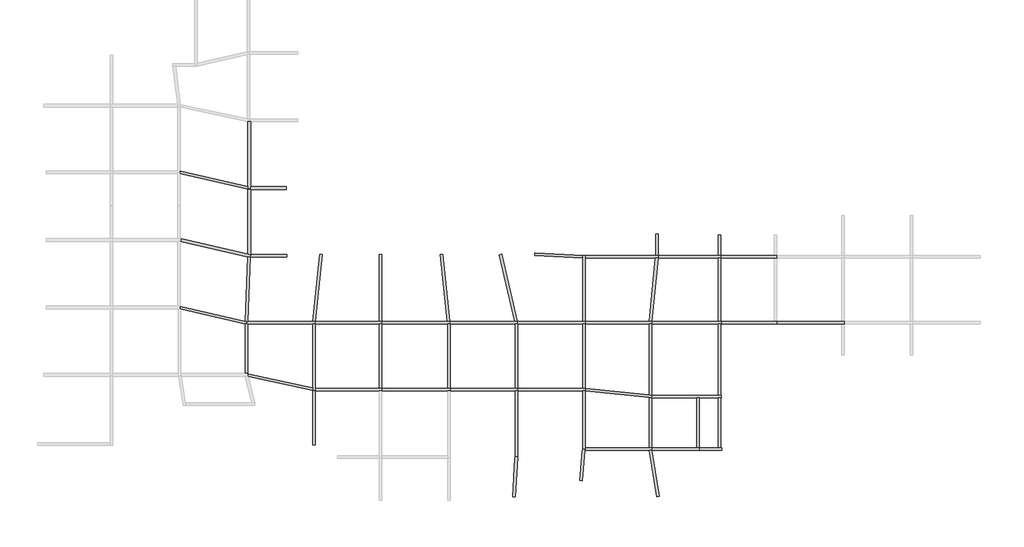
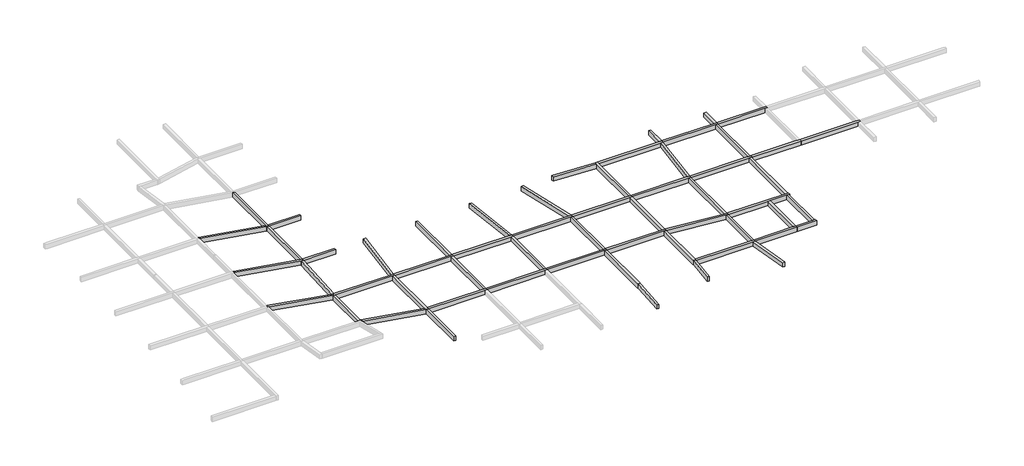
# One storey, part 4 of 8: 57 beams.
"""IFC4 building model written with IfcOpenShell, lengths in millimetres."""

from ifc_helpers import new_model, si_unit, frame, origin, place, context, project, spatial, polyline, outline, extrude, faceted_brep, element, save

model = new_model("IFC4")

# Units and contexts
model_context = context("Model", 3, world=origin())
ifc_project = project(units=[si_unit("LENGTHUNIT", "METRE", prefix="MILLI")], contexts=[model_context])

# Site, building, storey
site = spatial("IfcSite", under=ifc_project)
building = spatial("IfcBuilding", under=site)
storey = spatial("IfcBuildingStorey", under=building, Name="层高", Elevation=3300.0)

# Beams
placement = place(None, origin())
element("IfcBeam", 1, ObjectType="混凝土 - 矩形梁 : KL_beam", at=placement, inside=storey, context=model_context, shape_type="Brep", body=[
    faceted_brep([(165142.8646968, 66807.9309409, 3300.0), (165142.8646968, 59204.3834573, 3300.0), (165142.8646968, 58896.7990062, 3300.0), (165442.8646968, 58896.7990062, 3300.0), (165442.8646968, 59166.6493896, 3300.0), (165442.8646968, 66779.3985459, 3300.0), (165277.0990615, 66779.3985459, 3300.0), (165142.8646968, 66807.9309409, 2700.0), (165142.8646968, 59204.3834573, 2700.0), (165142.8646968, 58896.7990062, 2700.0), (165277.0990615, 66779.3985459, 2700.0), (165442.8646968, 66779.3985459, 2700.0), (165442.8646968, 59166.6493896, 2700.0), (165442.8646968, 58896.7990062, 2700.0)], [[[0, 1, 2, 3, 4, 5, 6]], [[2, 1, 0, 7, 8, 9]], [[9, 8, 7, 10, 11, 12, 13]], [[3, 13, 12, 11, 5, 4]], [[0, 6, 10, 7]], [[6, 5, 11, 10]], [[3, 2, 9, 13]]]),
])
element("IfcBeam", 2, ObjectType="混凝土 - 矩形梁 : KL_beam", at=placement, inside=storey, context=model_context, shape_type="SweptSolid", body=[
    extrude(outline(polyline([(165142.8646968, 58896.7990062), (157226.4248507, 60688.1226811), (157226.4248507, 60995.7071323), (165142.8646968, 59204.3834573), (165142.8646968, 58896.7990062)])), frame((0.0, 0.0, 2700.0), z_axis=(0.0, 0.0, 1.0), x_axis=(1.0, 0.0, 0.0)), (0.0, 0.0, 1.0), 600.0),
])
element("IfcBeam", 3, ObjectType="混凝土 - 矩形梁 : KL_beam", at=placement, inside=storey, context=model_context, shape_type="Brep", body=[
    faceted_brep([(169649.165188, 59166.6493896, 3300.0), (169649.165188, 58866.6493896, 3300.0), (169649.165188, 58866.6493896, 2700.0), (169649.165188, 59166.6493896, 2700.0), (165442.8646968, 59166.6493896, 3300.0), (165442.8646968, 59136.4997731, 3300.0), (165442.8646968, 58896.7990062, 3300.0), (165142.8646968, 58896.7990062, 3300.0), (165142.8646968, 58866.6493896, 3300.0), (165442.8646968, 58866.6493896, 3300.0), (165142.8646968, 58866.6493896, 2700.0), (165442.8646968, 58866.6493896, 2700.0), (165142.8646968, 58896.7990062, 2700.0), (165442.8646968, 58896.7990062, 2700.0), (165442.8646968, 59136.4997731, 2700.0), (165442.8646968, 59166.6493896, 2700.0)], [[[0, 1, 2, 3]], [[1, 0, 4, 5, 6, 7, 8, 9]], [[2, 1, 9, 8, 10, 11]], [[3, 2, 11, 10, 12, 13, 14, 15]], [[0, 3, 15, 4]], [[10, 8, 7, 12]], [[13, 6, 5, 4, 15, 14]], [[6, 13, 12, 7]]]),
])
element("IfcBeam", 4, ObjectType="混凝土 - 矩形梁 : KL_beam", at=placement, inside=storey, context=model_context, shape_type="Brep", body=[
    faceted_brep([(165375.3793805, 50905.9465121, 3300.0), (165380.6883405, 50928.942144, 3300.0), (165442.8646968, 51198.2575315, 3300.0), (165142.8646968, 51267.5179888, 3300.0), (157280.5913749, 53082.6668088, 3300.0), (157246.4106924, 52782.6668088, 3300.0), (165137.4631911, 50960.8737924, 3300.0), (165275.7743556, 50928.942144, 3300.0), (165375.3793805, 50905.9465121, 2700.0), (157246.4106924, 52782.6668088, 2700.0), (165137.4631911, 50960.8737924, 2700.0), (165275.7743556, 50928.942144, 2700.0), (165442.8646968, 51198.2575315, 2700.0), (165380.6883405, 50928.942144, 2700.0), (157280.5913749, 53082.6668088, 2700.0), (165142.8646968, 51267.5179888, 2700.0)], [[[0, 1, 2, 3, 4, 5, 6, 7]], [[8, 0, 7, 6, 5, 9, 10, 11]], [[12, 13, 8, 11, 10, 9, 14, 15]], [[2, 12, 15, 14, 4, 3]], [[2, 1, 0, 8, 13, 12]], [[4, 14, 9, 5]]]),
])
element("IfcBeam", 5, ObjectType="混凝土 - 矩形梁 : KL_beam", at=placement, inside=storey, context=model_context, shape_type="Brep", body=[
    faceted_brep([(165442.8646968, 58866.6493896, 3300.0), (165142.8646968, 58866.6493896, 3300.0), (165142.8646968, 51267.5179888, 3300.0), (165442.8646968, 51198.2575315, 3300.0), (165442.8646968, 51228.942144, 3300.0), (165142.8646968, 58866.6493896, 2700.0), (165142.8646968, 51267.5179888, 2700.0), (165442.8646968, 58866.6493896, 2700.0), (165442.8646968, 51228.942144, 2700.0), (165442.8646968, 51198.2575315, 2700.0)], [[[0, 1, 2, 3, 4]], [[1, 5, 6, 2]], [[5, 7, 8, 9, 6]], [[7, 0, 4, 3, 9, 8]], [[1, 0, 7, 5]], [[3, 2, 6, 9]]]),
])
element("IfcBeam", 6, ObjectType="混凝土 - 矩形梁 : KL_beam", at=placement, inside=storey, context=model_context, shape_type="Brep", body=[
    faceted_brep([(169692.8646968, 51228.942144, 3300.0), (169692.8646968, 50928.942144, 3300.0), (169692.8646968, 50928.942144, 2700.0), (169692.8646968, 51228.942144, 2700.0), (165442.8646968, 51228.942144, 3300.0), (165442.8646968, 51198.2575315, 3300.0), (165380.6883405, 50928.942144, 3300.0), (165436.3392696, 50928.942144, 3300.0), (165380.6883405, 50928.942144, 2700.0), (165436.3392696, 50928.942144, 2700.0), (165442.8646968, 51198.2575315, 2700.0), (165442.8646968, 51228.942144, 2700.0)], [[[0, 1, 2, 3]], [[1, 0, 4, 5, 6, 7]], [[2, 1, 7, 6, 8, 9]], [[3, 2, 9, 8, 10, 11]], [[0, 3, 11, 4]], [[6, 5, 10, 8]], [[5, 4, 11, 10]]]),
    faceted_brep([(165136.0424839, 50928.942144, 2700.0), (165136.0424839, 50928.942144, 3300.0), (165137.4631911, 50960.8737924, 3300.0), (165137.4631911, 50960.8737924, 2700.0), (165275.7743556, 50928.942144, 3300.0), (165275.7743556, 50928.942144, 2700.0), (165142.8646968, 50959.6267565, 2700.0), (165142.8646968, 50959.6267565, 3300.0)], [[[0, 1, 2, 3]], [[4, 5, 6, 3, 2, 7]], [[1, 4, 7, 2]], [[1, 0, 5, 4]], [[5, 0, 3, 6]]]),
])
element("IfcBeam", 7, ObjectType="混凝土 - 矩形梁 : KL_beam", at=placement, inside=storey, context=model_context, shape_type="Brep", body=[
    faceted_brep([(164960.8749274, 43383.0583741, 3300.0), (164801.942538, 43419.7508073, 3300.0), (157226.4248507, 45168.6968726, 3300.0), (157165.9144091, 45182.6668088, 3300.0), (157131.7337266, 44882.6668088, 3300.0), (157298.8240678, 44844.090964, 3300.0), (164793.7845861, 43113.7429866, 3300.0), (164926.6942449, 43083.0583741, 3300.0), (157131.7337266, 44882.6668088, 2700.0), (157298.8240678, 44844.090964, 2700.0), (164793.7845861, 43113.7429866, 2700.0), (164926.6942449, 43083.0583741, 2700.0), (157165.9144091, 45182.6668088, 2700.0), (157226.4248507, 45168.6968726, 2700.0), (164801.942538, 43419.7508073, 2700.0), (164960.8749274, 43383.0583741, 2700.0)], [[[0, 1, 2, 3, 4, 5, 6, 7]], [[7, 6, 5, 4, 8, 9, 10, 11]], [[11, 10, 9, 8, 12, 13, 14, 15]], [[3, 2, 1, 0, 15, 14, 13, 12]], [[3, 12, 8, 4]], [[0, 7, 11, 15]]]),
])
element("IfcBeam", 8, ObjectType="混凝土 - 矩形梁 : KL_beam", at=placement, inside=storey, context=model_context, shape_type="Brep", body=[
    faceted_brep([(164960.8749274, 43383.0583741, 3300.0), (164926.6942449, 43083.0583741, 3300.0), (165093.7845861, 43083.0583741, 3300.0), (172693.7845861, 43083.0583741, 3300.0), (172978.8451928, 43083.0583741, 3300.0), (173010.3764633, 43383.0583741, 3300.0), (172708.7239795, 43383.0583741, 3300.0), (165100.606799, 43383.0583741, 3300.0), (164926.6942449, 43083.0583741, 2700.0), (165093.7845861, 43083.0583741, 2700.0), (172693.7845861, 43083.0583741, 2700.0), (172978.8451928, 43083.0583741, 2700.0), (164960.8749274, 43383.0583741, 2700.0), (165100.606799, 43383.0583741, 2700.0), (172708.7239795, 43383.0583741, 2700.0), (173010.3764633, 43383.0583741, 2700.0)], [[[0, 1, 2, 3, 4, 5, 6, 7]], [[1, 8, 9, 10, 11, 4, 3, 2]], [[8, 12, 13, 14, 15, 11, 10, 9]], [[12, 0, 7, 6, 5, 15, 14, 13]], [[0, 12, 8, 1]], [[5, 4, 11, 15]]]),
])
element("IfcBeam", 9, ObjectType="混凝土 - 矩形梁 : KL_beam", at=placement, inside=storey, context=model_context, shape_type="SweptSolid", body=[
    extrude(outline(polyline([(165275.7743556, 50928.942144), (165375.3793805, 50905.9465121), (165380.6883405, 50928.942144), (165436.3392696, 50928.942144), (165100.606799, 43383.0583741), (164960.8749274, 43383.0583741), (164801.942538, 43419.7508073), (165136.0424839, 50928.942144), (165275.7743556, 50928.942144)])), frame((0.0, 0.0, 2700.0), z_axis=(0.0, 0.0, 1.0), x_axis=(1.0, 0.0, 0.0)), (0.0, 0.0, 1.0), 600.0),
])
element("IfcBeam", 10, ObjectType="混凝土 - 矩形梁 : KL_beam", at=placement, inside=storey, context=model_context, shape_type="SweptSolid", body=[
    extrude(outline(polyline([(173536.3056367, 51256.9718763), (173834.6622053, 51225.6133373), (173010.3764633, 43383.0583741), (172708.7239795, 43383.0583741), (173536.3056367, 51256.9718763)])), frame((0.0, 0.0, 2700.0), z_axis=(0.0, 0.0, 1.0), x_axis=(1.0, 0.0, 0.0)), (0.0, 0.0, 1.0), 600.0),
])
element("IfcBeam", 11, ObjectType="混凝土 - 矩形梁 : KL_beam", at=placement, inside=storey, context=model_context, shape_type="Brep", body=[
    faceted_brep([(173010.3764633, 43383.0583741, 3300.0), (172978.8451928, 43083.0583741, 3300.0), (172993.7845861, 43083.0583741, 3300.0), (180493.7845861, 43083.0583741, 3300.0), (180793.7845861, 43083.0583741, 3300.0), (180793.7845861, 43383.0583741, 3300.0), (180493.7845861, 43383.0583741, 3300.0), (172978.8451928, 43083.0583741, 2700.0), (172993.7845861, 43083.0583741, 2700.0), (180493.7845861, 43083.0583741, 2700.0), (180793.7845861, 43083.0583741, 2700.0), (173010.3764633, 43383.0583741, 2700.0), (180493.7845861, 43383.0583741, 2700.0), (180793.7845861, 43383.0583741, 2700.0)], [[[0, 1, 2, 3, 4, 5, 6]], [[1, 7, 8, 9, 10, 4, 3, 2]], [[7, 11, 12, 13, 10, 9, 8]], [[11, 0, 6, 5, 13, 12]], [[1, 0, 11, 7]], [[5, 4, 10, 13]]]),
])
element("IfcBeam", 12, ObjectType="混凝土 - 矩形梁 : KL_beam", at=placement, inside=storey, context=model_context, shape_type="Brep", body=[
    faceted_brep([(188778.8451928, 43083.0583741, 3300.0), (188778.8451928, 43383.0583741, 3300.0), (188477.1927089, 43383.0583741, 3300.0), (180793.7845861, 43383.0583741, 3300.0), (180793.7845861, 43083.0583741, 3300.0), (188493.7845861, 43083.0583741, 3300.0), (188778.8451928, 43083.0583741, 2700.0), (180793.7845861, 43083.0583741, 2700.0), (188493.7845861, 43083.0583741, 2700.0), (188778.8451928, 43383.0583741, 2700.0), (180793.7845861, 43383.0583741, 2700.0), (188477.1927089, 43383.0583741, 2700.0)], [[[0, 1, 2, 3, 4, 5]], [[6, 0, 5, 4, 7, 8]], [[9, 6, 8, 7, 10, 11]], [[1, 9, 11, 10, 3, 2]], [[1, 0, 6, 9]], [[4, 3, 10, 7]]]),
])
element("IfcBeam", 13, ObjectType="混凝土 - 矩形梁 : KL_beam", at=placement, inside=storey, context=model_context, shape_type="Brep", body=[
    faceted_brep([(196663.0999736, 43083.0583741, 3300.0), (196663.0999736, 43383.0583741, 3300.0), (196355.2087413, 43383.0583741, 3300.0), (188778.8451928, 43383.0583741, 3300.0), (188778.8451928, 43083.0583741, 3300.0), (188793.7845861, 43083.0583741, 3300.0), (196393.7845861, 43083.0583741, 3300.0), (196663.0999736, 43083.0583741, 2700.0), (188778.8451928, 43083.0583741, 2700.0), (188793.7845861, 43083.0583741, 2700.0), (196393.7845861, 43083.0583741, 2700.0), (196663.0999736, 43383.0583741, 2700.0), (188778.8451928, 43383.0583741, 2700.0), (196355.2087413, 43383.0583741, 2700.0)], [[[0, 1, 2, 3, 4, 5, 6]], [[7, 0, 6, 5, 4, 8, 9, 10]], [[11, 7, 10, 9, 8, 12, 13]], [[1, 11, 13, 12, 3, 2]], [[4, 3, 12, 8]], [[1, 0, 7, 11]]]),
])
element("IfcBeam", 14, ObjectType="混凝土 - 矩形梁 : KL_beam", at=placement, inside=storey, context=model_context, shape_type="Brep", body=[
    faceted_brep([(204593.7845861, 43083.0583741, 3300.0), (204593.7845861, 43383.0583741, 3300.0), (204293.7845861, 43383.0583741, 3300.0), (196663.0999736, 43383.0583741, 3300.0), (196663.0999736, 43083.0583741, 3300.0), (196693.7845861, 43083.0583741, 3300.0), (204293.7845861, 43083.0583741, 3300.0), (204593.7845861, 43083.0583741, 2700.0), (196663.0999736, 43083.0583741, 2700.0), (196693.7845861, 43083.0583741, 2700.0), (204293.7845861, 43083.0583741, 2700.0), (204593.7845861, 43383.0583741, 2700.0), (196663.0999736, 43383.0583741, 2700.0), (204293.7845861, 43383.0583741, 2700.0)], [[[0, 1, 2, 3, 4, 5, 6]], [[7, 0, 6, 5, 4, 8, 9, 10]], [[11, 7, 10, 9, 8, 12, 13]], [[1, 11, 13, 12, 3, 2]], [[4, 3, 12, 8]], [[1, 0, 7, 11]]]),
])
element("IfcBeam", 15, ObjectType="混凝土 - 矩形梁 : KL_beam", at=placement, inside=storey, context=model_context, shape_type="SweptSolid", body=[
    extrude(outline(polyline([(180493.7845861, 51241.347456), (180793.7845861, 51241.347456), (180793.7845861, 43383.0583741), (180493.7845861, 43383.0583741), (180493.7845861, 51241.347456)])), frame((0.0, 0.0, 2700.0), z_axis=(0.0, 0.0, 1.0), x_axis=(1.0, 0.0, 0.0)), (0.0, 0.0, 1.0), 600.0),
])
element("IfcBeam", 16, ObjectType="混凝土 - 矩形梁 : KL_beam", at=placement, inside=storey, context=model_context, shape_type="SweptSolid", body=[
    extrude(outline(polyline([(187652.906967, 51225.6133373), (187951.2635356, 51256.9718763), (188778.8451928, 43383.0583741), (188477.1927089, 43383.0583741), (187652.906967, 51225.6133373)])), frame((0.0, 0.0, 2700.0), z_axis=(0.0, 0.0, 1.0), x_axis=(1.0, 0.0, 0.0)), (0.0, 0.0, 1.0), 600.0),
])
element("IfcBeam", 17, ObjectType="混凝土 - 矩形梁 : KL_beam", at=placement, inside=storey, context=model_context, shape_type="SweptSolid", body=[
    extrude(outline(polyline([(194548.7297415, 51207.7785791), (194841.0407609, 51275.2638954), (196663.0999736, 43383.0583741), (196355.2087413, 43383.0583741), (194548.7297415, 51207.7785791)])), frame((0.0, 0.0, 2700.0), z_axis=(0.0, 0.0, 1.0), x_axis=(1.0, 0.0, 0.0)), (0.0, 0.0, 1.0), 600.0),
])
element("IfcBeam", 18, ObjectType="混凝土 - 矩形梁 : KL_beam", at=placement, inside=storey, context=model_context, shape_type="Brep", body=[
    faceted_brep([(204593.7845861, 51116.8475615, 3300.0), (204447.3701528, 51116.8475615, 3300.0), (204293.7845861, 51116.8475615, 3300.0), (204293.7845861, 50823.8512794, 3300.0), (204293.7845861, 43383.0583741, 3300.0), (204593.7845861, 43383.0583741, 3300.0), (204593.7845861, 50816.8475615, 3300.0), (204593.7845861, 51116.8475615, 2700.0), (204593.7845861, 43383.0583741, 2700.0), (204593.7845861, 50816.8475615, 2700.0), (204293.7845861, 51116.8475615, 2700.0), (204447.3701528, 51116.8475615, 2700.0), (204293.7845861, 43383.0583741, 2700.0), (204293.7845861, 50823.8512794, 2700.0)], [[[0, 1, 2, 3, 4, 5, 6]], [[7, 0, 6, 5, 8, 9]], [[10, 11, 7, 9, 8, 12, 13]], [[2, 10, 13, 12, 4, 3]], [[5, 4, 12, 8]], [[2, 1, 0, 7, 11, 10]]]),
])
element("IfcBeam", 19, ObjectType="混凝土 - 矩形梁 : KL_beam", at=placement, inside=storey, context=model_context, shape_type="Brep", body=[
    faceted_brep([(213148.824042, 50816.8475615, 3300.0), (213148.824042, 51116.8475615, 3300.0), (212848.824042, 51116.8475615, 3300.0), (204593.7845861, 51116.8475615, 3300.0), (204593.7845861, 50816.8475615, 3300.0), (212833.4665871, 50816.8475615, 3300.0), (213134.8928997, 50816.8475615, 3300.0), (213148.824042, 50816.8475615, 2700.0), (204593.7845861, 50816.8475615, 2700.0), (212833.4665871, 50816.8475615, 2700.0), (213134.8928997, 50816.8475615, 2700.0), (213148.824042, 51116.8475615, 2700.0), (204593.7845861, 51116.8475615, 2700.0), (212848.824042, 51116.8475615, 2700.0)], [[[0, 1, 2, 3, 4, 5, 6]], [[7, 0, 6, 5, 4, 8, 9, 10]], [[11, 7, 10, 9, 8, 12, 13]], [[1, 11, 13, 12, 3, 2]], [[1, 0, 7, 11]], [[4, 3, 12, 8]]]),
])
element("IfcBeam", 20, ObjectType="混凝土 - 矩形梁 : KL_beam", at=placement, inside=storey, context=model_context, shape_type="Brep", body=[
    faceted_brep([(220448.824042, 50816.8475615, 3300.0), (220448.824042, 51116.8475615, 3300.0), (220148.824042, 51116.8475615, 3300.0), (213148.824042, 51116.8475615, 3300.0), (213148.824042, 50816.8475615, 3300.0), (220148.824042, 50816.8475615, 3300.0), (220448.824042, 50816.8475615, 2700.0), (213148.824042, 50816.8475615, 2700.0), (220148.824042, 50816.8475615, 2700.0), (220448.824042, 51116.8475615, 2700.0), (213148.824042, 51116.8475615, 2700.0), (220148.824042, 51116.8475615, 2700.0)], [[[0, 1, 2, 3, 4, 5]], [[6, 0, 5, 4, 7, 8]], [[9, 6, 8, 7, 10, 11]], [[1, 9, 11, 10, 3, 2]], [[4, 3, 10, 7]], [[1, 0, 6, 9]]]),
])
element("IfcBeam", 21, ObjectType="混凝土 - 矩形梁 : KL_beam", at=placement, inside=storey, context=model_context, shape_type="Brep", body=[
    faceted_brep([(227048.824042, 50816.8475615, 3300.0), (227048.824042, 51116.8475615, 3300.0), (226748.824042, 51116.8475615, 3300.0), (220448.824042, 51116.8475615, 3300.0), (220448.824042, 50816.8475615, 3300.0), (226748.824042, 50816.8475615, 3300.0), (227048.824042, 50816.8475615, 2700.0), (220448.824042, 50816.8475615, 2700.0), (226748.824042, 50816.8475615, 2700.0), (227048.824042, 51116.8475615, 2700.0), (220448.824042, 51116.8475615, 2700.0), (226748.824042, 51116.8475615, 2700.0)], [[[0, 1, 2, 3, 4, 5]], [[6, 0, 5, 4, 7, 8]], [[9, 6, 8, 7, 10, 11]], [[1, 9, 11, 10, 3, 2]], [[4, 3, 10, 7]], [[1, 0, 6, 9]]]),
])
element("IfcBeam", 22, ObjectType="混凝土 - 矩形梁 : KL_beam", at=placement, inside=storey, context=model_context, shape_type="SweptSolid", body=[
    extrude(outline(polyline([(212848.824042, 53616.2422047), (213148.824042, 53616.2422047), (213148.824042, 51116.8475615), (212848.824042, 51116.8475615), (212848.824042, 53616.2422047)])), frame((0.0, 0.0, 2700.0), z_axis=(0.0, 0.0, 1.0), x_axis=(1.0, 0.0, 0.0)), (0.0, 0.0, 1.0), 600.0),
])
element("IfcBeam", 23, ObjectType="混凝土 - 矩形梁 : KL_beam", at=placement, inside=storey, context=model_context, shape_type="SweptSolid", body=[
    extrude(outline(polyline([(220148.824042, 53516.2415345), (220448.824042, 53516.2415345), (220448.824042, 51116.8475615), (220148.824042, 51116.8475615), (220148.824042, 53516.2415345)])), frame((0.0, 0.0, 2700.0), z_axis=(0.0, 0.0, 1.0), x_axis=(1.0, 0.0, 0.0)), (0.0, 0.0, 1.0), 600.0),
])
element("IfcBeam", 24, ObjectType="混凝土 - 矩形梁 : KL_beam", at=placement, inside=storey, context=model_context, shape_type="Brep", body=[
    faceted_brep([(164793.7845861, 43113.7429866, 3300.0), (164793.7845861, 43113.7429866, 2700.0), (164793.7845861, 37282.6668088, 2700.0), (164793.7845861, 37282.6668088, 3300.0), (164926.6942449, 43083.0583741, 3300.0), (164926.6942449, 43083.0583741, 2700.0), (165093.7845861, 43083.0583741, 3300.0), (165093.7845861, 43083.0583741, 2700.0), (165087.2591589, 43083.0583741, 2700.0), (165087.2591589, 43083.0583741, 3300.0), (165066.4046628, 37282.6668088, 2700.0), (165066.4046628, 37282.6668088, 3300.0), (165093.7845861, 37171.3323813, 2700.0), (165093.7845861, 37171.3323813, 3300.0), (165093.7845861, 37254.8965213, 3300.0), (165093.7845861, 37254.8965213, 2700.0)], [[[0, 1, 2, 3]], [[0, 4, 5, 1]], [[6, 7, 8, 5, 4, 9]], [[10, 11, 3, 2]], [[11, 10, 12, 13]], [[4, 0, 3, 11, 13, 14, 6, 9]], [[1, 5, 8, 7, 15, 12, 10, 2]], [[7, 6, 14, 13, 12, 15]]]),
])
element("IfcBeam", 25, ObjectType="混凝土 - 矩形梁 : KL_beam", at=placement, inside=storey, context=model_context, shape_type="Brep", body=[
    faceted_brep([(172993.7845861, 43083.0583741, 3300.0), (172978.8451928, 43083.0583741, 3300.0), (172693.7845861, 43083.0583741, 3300.0), (172693.7845861, 35618.7864895, 3300.0), (172693.7845861, 35311.9135493, 3300.0), (172693.7845861, 35283.0583741, 3300.0), (172827.8216176, 35283.0583741, 3300.0), (172993.7845861, 35283.0583741, 3300.0), (172993.7845861, 35583.0583741, 3300.0), (172693.7845861, 43083.0583741, 2700.0), (172693.7845861, 35618.7864895, 2700.0), (172693.7845861, 35311.9135493, 2700.0), (172693.7845861, 35283.0583741, 2700.0), (172978.8451928, 43083.0583741, 2700.0), (172993.7845861, 43083.0583741, 2700.0), (172993.7845861, 35583.0583741, 2700.0), (172993.7845861, 35283.0583741, 2700.0), (172827.8216176, 35283.0583741, 2700.0)], [[[0, 1, 2, 3, 4, 5, 6, 7, 8]], [[2, 9, 10, 11, 12, 5, 4, 3]], [[9, 13, 14, 15, 16, 17, 12, 11, 10]], [[7, 16, 15, 14, 0, 8]], [[0, 14, 13, 9, 2, 1]], [[7, 6, 5, 12, 17, 16]]]),
])
element("IfcBeam", 26, ObjectType="混凝土 - 矩形梁 : KL_beam", at=placement, inside=storey, context=model_context, shape_type="Brep", body=[
    faceted_brep([(180793.7845861, 35283.0583741, 3300.0), (180793.7845861, 35583.0583741, 3300.0), (180493.7845861, 35583.0583741, 3300.0), (172993.7845861, 35583.0583741, 3300.0), (172993.7845861, 35283.0583741, 3300.0), (180493.7845861, 35283.0583741, 3300.0), (180793.7845861, 35283.0583741, 2700.0), (172993.7845861, 35283.0583741, 2700.0), (180493.7845861, 35283.0583741, 2700.0), (180793.7845861, 35583.0583741, 2700.0), (172993.7845861, 35583.0583741, 2700.0), (180493.7845861, 35583.0583741, 2700.0)], [[[0, 1, 2, 3, 4, 5]], [[6, 0, 5, 4, 7, 8]], [[9, 6, 8, 7, 10, 11]], [[1, 9, 11, 10, 3, 2]], [[4, 3, 10, 7]], [[1, 0, 6, 9]]]),
])
element("IfcBeam", 27, ObjectType="混凝土 - 矩形梁 : KL_beam", at=placement, inside=storey, context=model_context, shape_type="Brep", body=[
    faceted_brep([(188793.7845861, 35283.0583741, 3300.0), (188793.7845861, 35583.0583741, 3300.0), (188493.7845861, 35583.0583741, 3300.0), (180793.7845861, 35583.0583741, 3300.0), (180793.7845861, 35283.0583741, 3300.0), (188493.7845861, 35283.0583741, 3300.0), (188793.7845861, 35283.0583741, 2700.0), (180793.7845861, 35283.0583741, 2700.0), (188493.7845861, 35283.0583741, 2700.0), (188793.7845861, 35583.0583741, 2700.0), (180793.7845861, 35583.0583741, 2700.0), (188493.7845861, 35583.0583741, 2700.0)], [[[0, 1, 2, 3, 4, 5]], [[6, 0, 5, 4, 7, 8]], [[9, 6, 8, 7, 10, 11]], [[1, 9, 11, 10, 3, 2]], [[4, 3, 10, 7]], [[1, 0, 6, 9]]]),
])
element("IfcBeam", 28, ObjectType="混凝土 - 矩形梁 : KL_beam", at=placement, inside=storey, context=model_context, shape_type="Brep", body=[
    faceted_brep([(196693.7845861, 35283.0583741, 3300.0), (196693.7845861, 35583.0583741, 3300.0), (196393.7845861, 35583.0583741, 3300.0), (188793.7845861, 35583.0583741, 3300.0), (188793.7845861, 35283.0583741, 3300.0), (196393.7845861, 35283.0583741, 3300.0), (196693.7845861, 35283.0583741, 2700.0), (188793.7845861, 35283.0583741, 2700.0), (196393.7845861, 35283.0583741, 2700.0), (196693.7845861, 35583.0583741, 2700.0), (188793.7845861, 35583.0583741, 2700.0), (196393.7845861, 35583.0583741, 2700.0)], [[[0, 1, 2, 3, 4, 5]], [[6, 0, 5, 4, 7, 8]], [[9, 6, 8, 7, 10, 11]], [[1, 9, 11, 10, 3, 2]], [[4, 3, 10, 7]], [[1, 0, 6, 9]]]),
])
element("IfcBeam", 29, ObjectType="混凝土 - 矩形梁 : KL_beam", at=placement, inside=storey, context=model_context, shape_type="Brep", body=[
    faceted_brep([(204593.7845861, 35283.0583741, 3300.0), (204593.7845861, 35568.1189807, 3300.0), (204593.7845861, 35583.0583741, 3300.0), (204293.7845861, 35583.0583741, 3300.0), (196693.7845861, 35583.0583741, 3300.0), (196693.7845861, 35283.0583741, 3300.0), (204293.7845861, 35283.0583741, 3300.0), (204593.7845861, 35283.0583741, 2700.0), (196693.7845861, 35283.0583741, 2700.0), (204293.7845861, 35283.0583741, 2700.0), (204593.7845861, 35583.0583741, 2700.0), (204593.7845861, 35568.1189807, 2700.0), (196693.7845861, 35583.0583741, 2700.0), (204293.7845861, 35583.0583741, 2700.0)], [[[0, 1, 2, 3, 4, 5, 6]], [[7, 0, 6, 5, 8, 9]], [[10, 11, 7, 9, 8, 12, 13]], [[2, 10, 13, 12, 4, 3]], [[5, 4, 12, 8]], [[2, 1, 0, 7, 11, 10]]]),
])
element("IfcBeam", 30, ObjectType="混凝土 - 矩形梁 : KL_beam", at=placement, inside=storey, context=model_context, shape_type="SweptSolid", body=[
    extrude(outline(polyline([(180493.7845861, 43083.0583741), (180793.7845861, 43083.0583741), (180793.7845861, 35583.0583741), (180493.7845861, 35583.0583741), (180493.7845861, 43083.0583741)])), frame((0.0, 0.0, 2700.0), z_axis=(0.0, 0.0, 1.0), x_axis=(1.0, 0.0, 0.0)), (0.0, 0.0, 1.0), 600.0),
])
element("IfcBeam", 31, ObjectType="混凝土 - 矩形梁 : KL_beam", at=placement, inside=storey, context=model_context, shape_type="Brep", body=[
    faceted_brep([(188793.7845861, 43083.0583741, 3300.0), (188778.8451928, 43083.0583741, 3300.0), (188493.7845861, 43083.0583741, 3300.0), (188493.7845861, 35583.0583741, 3300.0), (188793.7845861, 35583.0583741, 3300.0), (188493.7845861, 43083.0583741, 2700.0), (188493.7845861, 35583.0583741, 2700.0), (188778.8451928, 43083.0583741, 2700.0), (188793.7845861, 43083.0583741, 2700.0), (188793.7845861, 35583.0583741, 2700.0)], [[[0, 1, 2, 3, 4]], [[2, 5, 6, 3]], [[5, 7, 8, 9, 6]], [[8, 0, 4, 9]], [[5, 2, 1, 0, 8, 7]], [[4, 3, 6, 9]]]),
])
element("IfcBeam", 32, ObjectType="混凝土 - 矩形梁 : KL_beam", at=placement, inside=storey, context=model_context, shape_type="Brep", body=[
    faceted_brep([(196693.7845861, 43083.0583741, 3300.0), (196663.0999736, 43083.0583741, 3300.0), (196393.7845861, 43083.0583741, 3300.0), (196393.7845861, 35583.0583741, 3300.0), (196693.7845861, 35583.0583741, 3300.0), (196393.7845861, 43083.0583741, 2700.0), (196393.7845861, 35583.0583741, 2700.0), (196663.0999736, 43083.0583741, 2700.0), (196693.7845861, 43083.0583741, 2700.0), (196693.7845861, 35583.0583741, 2700.0)], [[[0, 1, 2, 3, 4]], [[2, 5, 6, 3]], [[5, 7, 8, 9, 6]], [[8, 0, 4, 9]], [[5, 2, 1, 0, 8, 7]], [[4, 3, 6, 9]]]),
])
element("IfcBeam", 33, ObjectType="混凝土 - 矩形梁 : KL_beam", at=placement, inside=storey, context=model_context, shape_type="SweptSolid", body=[
    extrude(outline(polyline([(204293.7845861, 43083.0583741), (204593.7845861, 43083.0583741), (204593.7845861, 35583.0583741), (204293.7845861, 35583.0583741), (204293.7845861, 43083.0583741)])), frame((0.0, 0.0, 2700.0), z_axis=(0.0, 0.0, 1.0), x_axis=(1.0, 0.0, 0.0)), (0.0, 0.0, 1.0), 600.0),
])
element("IfcBeam", 34, ObjectType="混凝土 - 矩形梁 : KL_beam", at=placement, inside=storey, context=model_context, shape_type="Brep", body=[
    faceted_brep([(172993.7845861, 35283.0583741, 3300.0), (172827.8216176, 35283.0583741, 3300.0), (172993.7845861, 35247.3302586, 3300.0), (172827.8216176, 35283.0583741, 2700.0), (172993.7845861, 35247.3302586, 2700.0), (172993.7845861, 35283.0583741, 2700.0)], [[[0, 1, 2]], [[1, 3, 4, 2]], [[3, 5, 4]], [[5, 0, 2, 4]], [[1, 0, 5, 3]]]),
    faceted_brep([(172693.7845861, 35618.7864895, 3300.0), (172693.7845861, 35618.7864895, 2700.0), (165093.7845861, 37254.8965213, 2700.0), (165093.7845861, 37254.8965213, 3300.0), (165151.7717786, 36935.5402354, 2700.0), (165151.7717786, 36935.5402354, 3300.0), (165140.1821742, 36982.6668088, 3300.0), (165093.7845861, 37171.3323813, 3300.0), (165093.7845861, 37171.3323813, 2700.0), (165140.1821742, 36982.6668088, 2700.0), (172693.7845861, 35311.9135493, 3300.0), (172693.7845861, 35311.9135493, 2700.0), (172693.7845861, 35583.0583741, 2700.0), (172693.7845861, 35583.0583741, 3300.0)], [[[0, 1, 2, 3]], [[4, 5, 6, 7, 8, 9]], [[10, 11, 12, 1, 0, 13]], [[3, 2, 8, 7]], [[5, 10, 13, 0, 3, 7, 6]], [[5, 4, 11, 10]], [[11, 4, 9, 8, 2, 1, 12]]]),
])
element("IfcBeam", 35, ObjectType="混凝土 - 矩形梁 : KL_beam", at=placement, inside=storey, context=model_context, shape_type="SweptSolid", body=[
    extrude(outline(polyline([(172993.7845861, 28970.8720205), (172693.7845861, 28970.8720205), (172693.7845861, 35283.0583741), (172827.8216176, 35283.0583741), (172993.7845861, 35247.3302586), (172993.7845861, 28970.8720205)])), frame((0.0, 0.0, 2700.0), z_axis=(0.0, 0.0, 1.0), x_axis=(1.0, 0.0, 0.0)), (0.0, 0.0, 1.0), 600.0),
])
element("IfcBeam", 36, ObjectType="混凝土 - 矩形梁 : KL_beam", at=placement, inside=storey, context=model_context, shape_type="Brep", body=[
    faceted_brep([(196393.7845861, 27536.9862623, 3300.0), (196693.7845861, 27529.1304858, 3300.0), (196693.7845861, 27701.1172453, 3300.0), (196693.7845861, 35283.0583741, 3300.0), (196393.7845861, 35283.0583741, 3300.0), (196393.7845861, 27683.0583741, 3300.0), (196393.7845861, 27536.9862623, 2700.0), (196393.7845861, 35283.0583741, 2700.0), (196393.7845861, 27683.0583741, 2700.0), (196693.7845861, 27529.1304858, 2700.0), (196693.7845861, 35283.0583741, 2700.0), (196693.7845861, 27701.1172453, 2700.0)], [[[0, 1, 2, 3, 4, 5]], [[6, 0, 5, 4, 7, 8]], [[9, 6, 8, 7, 10, 11]], [[1, 9, 11, 10, 3, 2]], [[4, 3, 10, 7]], [[1, 0, 6, 9]]]),
])
element("IfcBeam", 37, ObjectType="混凝土 - 矩形梁 : KL_beam", at=placement, inside=storey, context=model_context, shape_type="Brep", body=[
    faceted_brep([(204293.7845861, 28439.6075155, 3300.0), (204593.7845861, 28426.5092326, 3300.0), (204593.7845861, 28583.0583741, 3300.0), (204593.7845861, 35266.4664969, 3300.0), (204593.7845861, 35283.0583741, 3300.0), (204293.7845861, 35283.0583741, 3300.0), (204293.7845861, 28566.9400301, 3300.0), (204293.7845861, 28439.6075155, 2700.0), (204293.7845861, 35283.0583741, 2700.0), (204293.7845861, 28566.9400301, 2700.0), (204593.7845861, 28426.5092326, 2700.0), (204593.7845861, 35283.0583741, 2700.0), (204593.7845861, 35266.4664969, 2700.0), (204593.7845861, 28583.0583741, 2700.0)], [[[0, 1, 2, 3, 4, 5, 6]], [[7, 0, 6, 5, 8, 9]], [[10, 7, 9, 8, 11, 12, 13]], [[1, 10, 13, 12, 11, 4, 3, 2]], [[5, 4, 11, 8]], [[1, 0, 7, 10]]]),
])
element("IfcBeam", 38, ObjectType="混凝土 - 矩形梁 : KL_beam", at=placement, inside=storey, context=model_context, shape_type="Brep", body=[
    faceted_brep([(212379.8534438, 43083.0583741, 3300.0), (212409.142041, 43383.0583741, 3300.0), (212107.7157284, 43383.0583741, 3300.0), (204593.7845861, 43383.0583741, 3300.0), (204593.7845861, 43083.0583741, 3300.0), (212093.7845861, 43083.0583741, 3300.0), (212379.8534438, 43083.0583741, 2700.0), (204593.7845861, 43083.0583741, 2700.0), (212093.7845861, 43083.0583741, 2700.0), (212409.142041, 43383.0583741, 2700.0), (204593.7845861, 43383.0583741, 2700.0), (212107.7157284, 43383.0583741, 2700.0)], [[[0, 1, 2, 3, 4, 5]], [[6, 0, 5, 4, 7, 8]], [[9, 6, 8, 7, 10, 11]], [[1, 9, 11, 10, 3, 2]], [[4, 3, 10, 7]], [[1, 0, 6, 9]]]),
])
element("IfcBeam", 39, ObjectType="混凝土 - 矩形梁 : KL_beam", at=placement, inside=storey, context=model_context, shape_type="Brep", body=[
    faceted_brep([(212833.4665871, 50816.8475615, 3300.0), (212833.4665871, 50816.8475615, 2700.0), (212107.7157284, 43383.0583741, 2700.0), (212107.7157284, 43383.0583741, 3300.0), (213134.8928997, 50816.8475615, 3300.0), (213134.8928997, 50816.8475615, 2700.0), (212848.824042, 50816.8475615, 2700.0), (212848.824042, 50816.8475615, 3300.0), (212409.142041, 43383.0583741, 3300.0), (212409.142041, 43383.0583741, 2700.0)], [[[0, 1, 2, 3]], [[4, 5, 6, 1, 0, 7]], [[7, 0, 3, 8, 4]], [[5, 4, 8, 9]], [[6, 5, 9, 2, 1]], [[3, 2, 9, 8]]]),
])
element("IfcBeam", 40, ObjectType="混凝土 - 矩形梁 : KL_beam", at=placement, inside=storey, context=model_context, shape_type="Brep", body=[
    faceted_brep([(220543.7845861, 43383.0583741, 3300.0), (220543.7845861, 43083.0583741, 3300.0), (220543.7845861, 43083.0583741, 2700.0), (220543.7845861, 43383.0583741, 2700.0), (220448.824042, 43383.0583741, 3300.0), (220148.824042, 43383.0583741, 3300.0), (212409.142041, 43383.0583741, 3300.0), (212379.8534438, 43083.0583741, 3300.0), (212393.7845861, 43083.0583741, 3300.0), (220148.824042, 43083.0583741, 3300.0), (220448.824042, 43083.0583741, 3300.0), (212379.8534438, 43083.0583741, 2700.0), (212393.7845861, 43083.0583741, 2700.0), (220148.824042, 43083.0583741, 2700.0), (220448.824042, 43083.0583741, 2700.0), (212409.142041, 43383.0583741, 2700.0), (220148.824042, 43383.0583741, 2700.0), (220448.824042, 43383.0583741, 2700.0)], [[[0, 1, 2, 3]], [[1, 0, 4, 5, 6, 7, 8, 9, 10]], [[2, 1, 10, 9, 8, 7, 11, 12, 13, 14]], [[3, 2, 14, 13, 12, 11, 15, 16, 17]], [[0, 3, 17, 16, 15, 6, 5, 4]], [[7, 6, 15, 11]]]),
])
element("IfcBeam", 41, ObjectType="混凝土 - 矩形梁 : KL_beam", at=placement, inside=storey, context=model_context, shape_type="SweptSolid", body=[
    extrude(outline(polyline([(220148.824042, 50816.8475615), (220448.824042, 50816.8475615), (220448.824042, 43383.0583741), (220148.824042, 43383.0583741), (220148.824042, 50816.8475615)])), frame((0.0, 0.0, 2700.0), z_axis=(0.0, 0.0, 1.0), x_axis=(1.0, 0.0, 0.0)), (0.0, 0.0, 1.0), 600.0),
])
element("IfcBeam", 42, ObjectType="混凝土 - 矩形梁 : KL_beam", at=placement, inside=storey, context=model_context, shape_type="Brep", body=[
    faceted_brep([(212393.7845861, 34748.3059456, 3300.0), (212093.7845861, 34779.8372162, 3300.0), (204593.7845861, 35568.1189807, 3300.0), (204593.7845861, 35283.0583741, 3300.0), (204593.7845861, 35266.4664969, 3300.0), (212093.7845861, 34478.1847324, 3300.0), (212235.9234192, 34463.245339, 3300.0), (212362.4260471, 34449.949377, 3300.0), (212363.8235091, 34463.245339, 3300.0), (212362.4260471, 34449.949377, 2700.0), (204593.7845861, 35266.4664969, 2700.0), (212093.7845861, 34478.1847324, 2700.0), (212235.9234192, 34463.245339, 2700.0), (204593.7845861, 35283.0583741, 2700.0), (204593.7845861, 35568.1189807, 2700.0), (212093.7845861, 34779.8372162, 2700.0), (212393.7845861, 34748.3059456, 2700.0), (212363.8235091, 34463.245339, 2700.0)], [[[0, 1, 2, 3, 4, 5, 6, 7, 8]], [[9, 7, 6, 5, 4, 10, 11, 12]], [[10, 13, 14, 15, 16, 17, 9, 12, 11]], [[2, 1, 0, 16, 15, 14]], [[2, 14, 13, 10, 4, 3]], [[0, 8, 7, 9, 17, 16]]]),
])
element("IfcBeam", 43, ObjectType="混凝土 - 矩形梁 : KL_beam", at=placement, inside=storey, context=model_context, shape_type="Brep", body=[
    faceted_brep([(212393.7845861, 34748.3059456, 3300.0), (212393.7845861, 34763.245339, 3300.0), (212393.7845861, 43083.0583741, 3300.0), (212379.8534438, 43083.0583741, 3300.0), (212093.7845861, 43083.0583741, 3300.0), (212093.7845861, 34779.8372162, 3300.0), (212093.7845861, 43083.0583741, 2700.0), (212093.7845861, 34779.8372162, 2700.0), (212393.7845861, 43083.0583741, 2700.0), (212393.7845861, 34763.245339, 2700.0), (212393.7845861, 34748.3059456, 2700.0), (212379.8534438, 43083.0583741, 2700.0)], [[[0, 1, 2, 3, 4, 5]], [[4, 6, 7, 5]], [[8, 9, 10, 7, 6, 11]], [[2, 1, 0, 10, 9, 8]], [[6, 4, 3, 2, 8, 11]], [[0, 5, 7, 10]]]),
])
element("IfcBeam", 44, ObjectType="混凝土 - 矩形梁 : KL_beam", at=placement, inside=storey, context=model_context, shape_type="Brep", body=[
    faceted_brep([(220543.7845861, 34763.245339, 3300.0), (220543.7845861, 34463.245339, 3300.0), (220543.7845861, 34463.245339, 2700.0), (220543.7845861, 34763.245339, 2700.0), (220448.824042, 34763.245339, 3300.0), (220148.824042, 34763.245339, 3300.0), (212393.7845861, 34763.245339, 3300.0), (212393.7845861, 34748.3059456, 3300.0), (212363.8235091, 34463.245339, 3300.0), (212393.7845861, 34463.245339, 3300.0), (217674.1922923, 34463.245339, 3300.0), (217974.1922923, 34463.245339, 3300.0), (220148.824042, 34463.245339, 3300.0), (220448.824042, 34463.245339, 3300.0), (212363.8235091, 34463.245339, 2700.0), (212393.7845861, 34463.245339, 2700.0), (217674.1922923, 34463.245339, 2700.0), (217974.1922923, 34463.245339, 2700.0), (220148.824042, 34463.245339, 2700.0), (220448.824042, 34463.245339, 2700.0), (212393.7845861, 34748.3059456, 2700.0), (212393.7845861, 34763.245339, 2700.0), (220148.824042, 34763.245339, 2700.0), (220448.824042, 34763.245339, 2700.0)], [[[0, 1, 2, 3]], [[1, 0, 4, 5, 6, 7, 8, 9, 10, 11, 12, 13]], [[2, 1, 13, 12, 11, 10, 9, 8, 14, 15, 16, 17, 18, 19]], [[3, 2, 19, 18, 17, 16, 15, 14, 20, 21, 22, 23]], [[0, 3, 23, 22, 21, 6, 5, 4]], [[8, 7, 20, 14]], [[7, 6, 21, 20]]]),
    faceted_brep([(212093.7845861, 34463.245339, 2700.0), (212093.7845861, 34463.245339, 3300.0), (212093.7845861, 34478.1847324, 3300.0), (212093.7845861, 34478.1847324, 2700.0), (212235.9234192, 34463.245339, 3300.0), (212235.9234192, 34463.245339, 2700.0)], [[[0, 1, 2, 3]], [[2, 4, 5, 3]], [[1, 4, 2]], [[1, 0, 5, 4]], [[5, 0, 3]]]),
])
element("IfcBeam", 45, ObjectType="混凝土 - 矩形梁 : KL_beam", at=placement, inside=storey, context=model_context, shape_type="SweptSolid", body=[
    extrude(outline(polyline([(220148.824042, 43083.0583741), (220448.824042, 43083.0583741), (220448.824042, 34763.245339), (220148.824042, 34763.245339), (220148.824042, 43083.0583741)])), frame((0.0, 0.0, 2700.0), z_axis=(0.0, 0.0, 1.0), x_axis=(1.0, 0.0, 0.0)), (0.0, 0.0, 1.0), 600.0),
])
element("IfcBeam", 46, ObjectType="混凝土 - 矩形梁 : KL_beam", at=placement, inside=storey, context=model_context, shape_type="Brep", body=[
    faceted_brep([(227048.824042, 43083.0583741, 3300.0), (227048.824042, 43383.0583741, 3300.0), (226748.824042, 43383.0583741, 3300.0), (220543.7845861, 43383.0583741, 3300.0), (220543.7845861, 43083.0583741, 3300.0), (227048.824042, 43083.0583741, 2700.0), (220543.7845861, 43083.0583741, 2700.0), (227048.824042, 43383.0583741, 2700.0), (220543.7845861, 43383.0583741, 2700.0), (226748.824042, 43383.0583741, 2700.0)], [[[0, 1, 2, 3, 4]], [[5, 0, 4, 6]], [[7, 5, 6, 8, 9]], [[1, 7, 9, 8, 3, 2]], [[4, 3, 8, 6]], [[1, 0, 5, 7]]]),
])
element("IfcBeam", 47, ObjectType="混凝土 - 矩形梁 : KL_beam", at=placement, inside=storey, context=model_context, shape_type="Brep", body=[
    faceted_brep([(234948.824042, 43083.0583741, 3300.0), (234948.824042, 43383.0583741, 3300.0), (234648.824042, 43383.0583741, 3300.0), (227048.824042, 43383.0583741, 3300.0), (227048.824042, 43083.0583741, 3300.0), (234648.824042, 43083.0583741, 3300.0), (234948.824042, 43083.0583741, 2700.0), (227048.824042, 43083.0583741, 2700.0), (234648.824042, 43083.0583741, 2700.0), (234948.824042, 43383.0583741, 2700.0), (227048.824042, 43383.0583741, 2700.0), (234648.824042, 43383.0583741, 2700.0)], [[[0, 1, 2, 3, 4, 5]], [[6, 0, 5, 4, 7, 8]], [[9, 6, 8, 7, 10, 11]], [[1, 9, 11, 10, 3, 2]], [[4, 3, 10, 7]], [[1, 0, 6, 9]]]),
])
element("IfcBeam", 48, ObjectType="混凝土 - 矩形梁 : KL_beam", at=placement, inside=storey, context=model_context, shape_type="Brep", body=[
    faceted_brep([(204270.7375427, 24734.0646297, 3300.0), (203971.8791332, 24760.2113525, 3300.0), (203971.8791332, 24760.2113525, 2700.0), (204270.7375427, 24734.0646297, 2700.0), (204581.2342622, 28283.0583741, 3300.0), (204593.7845861, 28426.5092326, 3300.0), (204293.7845861, 28439.6075155, 3300.0), (204278.3545725, 28263.2416532, 3300.0), (204293.7845861, 28439.6075155, 2700.0), (204278.3545725, 28263.2416532, 2700.0), (204593.7845861, 28426.5092326, 2700.0), (204581.2342622, 28283.0583741, 2700.0)], [[[0, 1, 2, 3]], [[1, 0, 4, 5, 6, 7]], [[2, 1, 7, 6, 8, 9]], [[3, 2, 9, 8, 10, 11]], [[0, 3, 11, 10, 5, 4]], [[5, 10, 8, 6]]]),
])
element("IfcBeam", 49, ObjectType="混凝土 - 矩形梁 : KL_beam", at=placement, inside=storey, context=model_context, shape_type="Brep", body=[
    faceted_brep([(204593.7845861, 28583.0583741, 3300.0), (204593.7845861, 28426.5092326, 3300.0), (204581.2342622, 28283.0583741, 3300.0), (212115.6724833, 28283.0583741, 3300.0), (212393.7845861, 28283.0583741, 3300.0), (212393.7845861, 28583.0583741, 3300.0), (212093.7845861, 28583.0583741, 3300.0), (212393.7845861, 28283.0583741, 2700.0), (204581.2342622, 28283.0583741, 2700.0), (212115.6724833, 28283.0583741, 2700.0), (204593.7845861, 28426.5092326, 2700.0), (204593.7845861, 28583.0583741, 2700.0), (212093.7845861, 28583.0583741, 2700.0), (212393.7845861, 28583.0583741, 2700.0)], [[[0, 1, 2, 3, 4, 5, 6]], [[7, 4, 3, 2, 8, 9]], [[10, 11, 12, 13, 7, 9, 8]], [[11, 0, 6, 5, 13, 12]], [[1, 0, 11, 10]], [[2, 1, 10, 8]], [[5, 4, 7, 13]]]),
])
element("IfcBeam", 50, ObjectType="混凝土 - 矩形梁 : KL_beam", at=placement, inside=storey, context=model_context, shape_type="SweptSolid", body=[
    extrude(outline(polyline([(212235.9234192, 34463.245339), (212362.4260471, 34449.949377), (212363.8235091, 34463.245339), (212393.7845861, 34463.245339), (212393.7845861, 28583.0583741), (212093.7845861, 28583.0583741), (212093.7845861, 34463.245339), (212235.9234192, 34463.245339)])), frame((0.0, 0.0, 2700.0), z_axis=(0.0, 0.0, 1.0), x_axis=(1.0, 0.0, 0.0)), (0.0, 0.0, 1.0), 600.0),
])
element("IfcBeam", 51, ObjectType="混凝土 - 矩形梁 : KL_beam", at=placement, inside=storey, context=model_context, shape_type="Brep", body=[
    faceted_brep([(217974.1922923, 28283.0583741, 3300.0), (217974.1922923, 28583.0583741, 3300.0), (217674.1922923, 28583.0583741, 3300.0), (212393.7845861, 28583.0583741, 3300.0), (212393.7845861, 28283.0583741, 3300.0), (212419.412021, 28283.0583741, 3300.0), (217974.1922923, 28283.0583741, 2700.0), (212393.7845861, 28283.0583741, 2700.0), (212419.412021, 28283.0583741, 2700.0), (217974.1922923, 28583.0583741, 2700.0), (212393.7845861, 28583.0583741, 2700.0), (217674.1922923, 28583.0583741, 2700.0)], [[[0, 1, 2, 3, 4, 5]], [[6, 0, 5, 4, 7, 8]], [[9, 6, 8, 7, 10, 11]], [[1, 9, 11, 10, 3, 2]], [[4, 3, 10, 7]], [[1, 0, 6, 9]]]),
])
element("IfcBeam", 52, ObjectType="混凝土 - 矩形梁 : KL_beam", at=placement, inside=storey, context=model_context, shape_type="Brep", body=[
    faceted_brep([(220574.2714263, 28583.0583741, 3300.0), (220574.2714263, 28283.0583741, 3300.0), (220574.2714263, 28283.0583741, 2700.0), (220574.2714263, 28583.0583741, 2700.0), (220448.824042, 28583.0583741, 3300.0), (220148.824042, 28583.0583741, 3300.0), (217974.1922923, 28583.0583741, 3300.0), (217974.1922923, 28283.0583741, 3300.0), (217974.1922923, 28283.0583741, 2700.0), (217974.1922923, 28583.0583741, 2700.0), (220148.824042, 28583.0583741, 2700.0), (220448.824042, 28583.0583741, 2700.0)], [[[0, 1, 2, 3]], [[1, 0, 4, 5, 6, 7]], [[2, 1, 7, 8]], [[3, 2, 8, 9, 10, 11]], [[0, 3, 11, 10, 9, 6, 5, 4]], [[7, 6, 9, 8]]]),
])
element("IfcBeam", 53, ObjectType="混凝土 - 矩形梁 : KL_beam", at=placement, inside=storey, context=model_context, shape_type="SweptSolid", body=[
    extrude(outline(polyline([(217974.1922923, 28583.0583741), (217674.1922923, 28583.0583741), (217674.1922923, 34463.245339), (217974.1922923, 34463.245339), (217974.1922923, 28583.0583741)])), frame((0.0, 0.0, 2700.0), z_axis=(0.0, 0.0, 1.0), x_axis=(1.0, 0.0, 0.0)), (0.0, 0.0, 1.0), 600.0),
])
element("IfcBeam", 54, ObjectType="混凝土 - 矩形梁 : KL_beam", at=placement, inside=storey, context=model_context, shape_type="SweptSolid", body=[
    extrude(outline(polyline([(220148.824042, 34463.245339), (220448.824042, 34463.245339), (220448.824042, 28583.0583741), (220148.824042, 28583.0583741), (220148.824042, 34463.245339)])), frame((0.0, 0.0, 2700.0), z_axis=(0.0, 0.0, 1.0), x_axis=(1.0, 0.0, 0.0)), (0.0, 0.0, 1.0), 600.0),
])
element("IfcBeam", 55, ObjectType="混凝土 - 矩形梁 : KL_beam", at=placement, inside=storey, context=model_context, shape_type="Brep", body=[
    faceted_brep([(213267.378499, 22929.2087396, 3300.0), (212971.0719968, 22882.2784001, 3300.0), (212971.0719968, 22882.2784001, 2700.0), (213267.378499, 22929.2087396, 2700.0), (212419.412021, 28283.0583741, 3300.0), (212393.7845861, 28283.0583741, 3300.0), (212115.6724833, 28283.0583741, 3300.0), (212115.6724833, 28283.0583741, 2700.0), (212393.7845861, 28283.0583741, 2700.0), (212419.412021, 28283.0583741, 2700.0)], [[[0, 1, 2, 3]], [[1, 0, 4, 5, 6]], [[2, 1, 6, 7]], [[3, 2, 7, 8, 9]], [[0, 3, 9, 4]], [[4, 9, 8, 7, 6, 5]]]),
])
element("IfcBeam", 56, ObjectType="混凝土 - 矩形梁 : KL_beam", at=placement, inside=storey, context=model_context, shape_type="Brep", body=[
    faceted_brep([(196447.600022, 22831.6491673, 3300.0), (196148.0111616, 22847.3499542, 3300.0), (196148.0111616, 22847.3499542, 2700.0), (196447.600022, 22831.6491673, 2700.0), (196686.9330908, 27398.3961679, 3300.0), (196693.7845861, 27529.1304858, 3300.0), (196393.7845861, 27536.9862623, 3300.0), (196385.7175673, 27383.0583741, 3300.0), (196393.7845861, 27536.9862623, 2700.0), (196385.7175673, 27383.0583741, 2700.0), (196693.7845861, 27529.1304858, 2700.0), (196686.9330908, 27398.3961679, 2700.0)], [[[0, 1, 2, 3]], [[1, 0, 4, 5, 6, 7]], [[2, 1, 7, 6, 8, 9]], [[3, 2, 9, 8, 10, 11]], [[0, 3, 11, 10, 5, 4]], [[5, 10, 8, 6]]]),
])
element("IfcBeam", 57, ObjectType="混凝土 - 矩形梁 : KL_beam", at=placement, inside=storey, context=model_context, shape_type="SweptSolid", body=[
    extrude(outline(polyline([(198692.136428, 51091.8054894), (198706.4705042, 51391.4628508), (204447.3701528, 51116.8475615), (204293.7845861, 51116.8475615), (204293.7845861, 50823.8512794), (198692.136428, 51091.8054894)])), frame((0.0, 0.0, 2700.0), z_axis=(0.0, 0.0, 1.0), x_axis=(1.0, 0.0, 0.0)), (0.0, 0.0, 1.0), 600.0),
])

save(model, "model.ifc")

# Revit data of these elements
# Type "混凝土 - 矩形梁 : KL_beam"
#   Length [instance default] = 1524 mm
#   b = 300 mm
#   h = 600 mm
#   Structural Material [instance default] = 混凝土 - 现场浇注混凝土
#   Assembly Code = ""
# Elements 1, 2, 3, 4, 5, 6, 7, 8, 9, 10, 11, 12, 13, 14, 15, 16, 17, 18, 19, 20, 21, 22, 23, 24, 25, 26, 27, 28, 29, 30, 31, 32, 33, 34, 35, 36, 37, 38, 39, 40, 41, 42, 43, 44, 45, 46, 47, 48, 49, 50, 51, 52, 53, 54, 55, 56, 57 (IfcBeam, "混凝土 - 矩形梁 : KL_beam")
#   Comments = ""
#   Structural Material = none
#   Phase Created = 新构造
# Materials
#   "混凝土 - 现场浇注混凝土": class "混凝土", colour RGB 192 192 192, transparency 0
